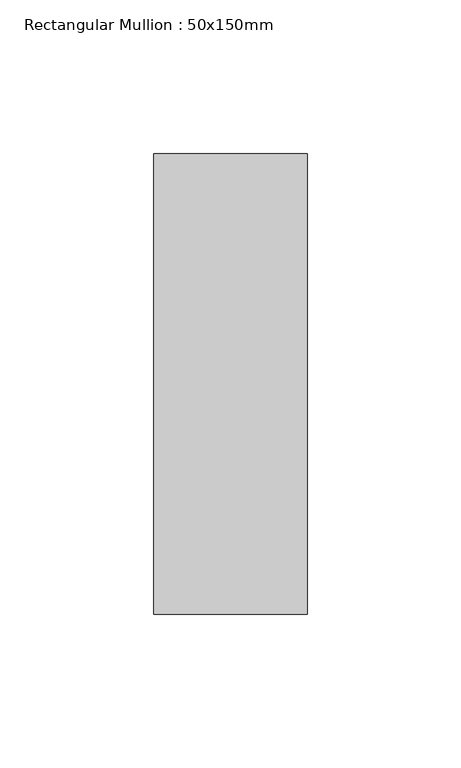
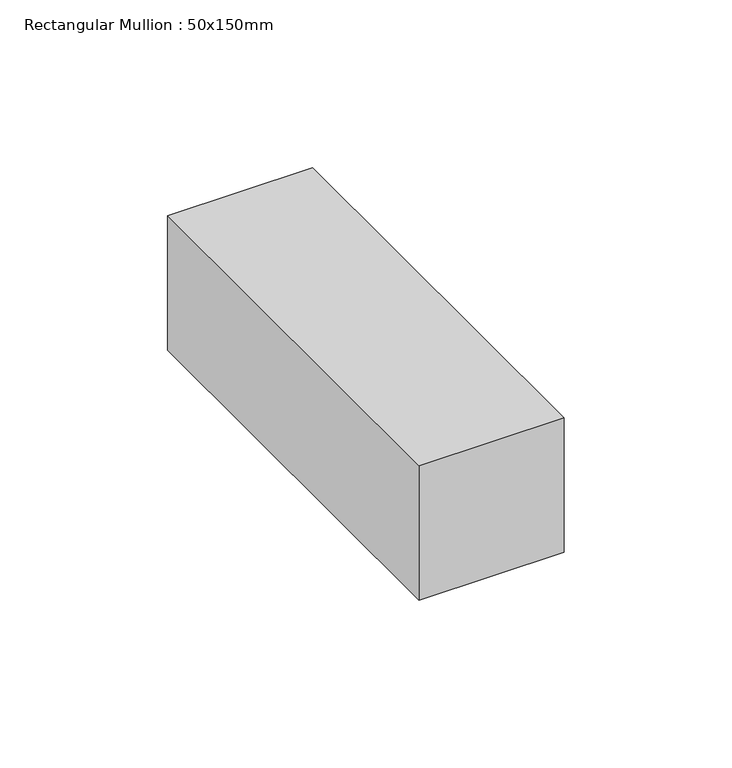
"""IFC4 building model written with IfcOpenShell, lengths in millimetres: member geometry, Rectangular Mullion : 50x150mm."""

from ifc_helpers import new_model, si_unit, frame, origin, place, context, project, spatial, polyline, outline, extrude, source, transform, mapped, element, save


def rectangular_mullion_50x150mm_fbc2abbf(model_context):
    return source(origin(), model_context, "Body", "SweptSolid", [
        extrude(outline(polyline([(25.0, 75.0), (25.0, -75.0), (-25.0, -75.0), (-25.0, 75.0), (25.0, 75.0)])), frame((0.0, 0.0, -49.0185145), z_axis=(0.0, 0.0, 1.0), x_axis=(1.0, 0.0, 0.0)), (0.0, 0.0, 1.0), 49.0185145),
    ])


if __name__ == "__main__":
    model = new_model("IFC4")
    model_context = context("Model", 3, world=origin())
    ifc_project = project(units=[si_unit("LENGTHUNIT", "METRE", prefix="MILLI")], contexts=[model_context])
    site = spatial("IfcSite", under=ifc_project)
    building = spatial("IfcBuilding", under=site)
    placement = place(None, origin())
    rectangular_mullion_50x150mm_shape = rectangular_mullion_50x150mm_fbc2abbf(model_context)
    element("IfcMember", 1, ObjectType="Rectangular Mullion : 50x150mm", at=placement, inside=building, context=model_context, shape_type="MappedRepresentation", body=[
        mapped(rectangular_mullion_50x150mm_shape, transform((0.0, 0.0, 0.0), x_axis=(1.0, 0.0, 0.0), y_axis=(0.0, 1.0, 0.0), z_axis=(0.0, 0.0, 1.0))),
    ])
    save(model, "model.ifc")

# Revit data of these elements
# Type "Rectangular Mullion : 50x150mm"
#   Keynote = "H11"
#   built-in parameter 1007304 = 0.492126 (stored number, unit not read)
#   built-in parameter 1007301 = 0.082021 (stored number, unit not read)
#   built-in parameter 1007300 = 0.082021 (stored number, unit not read)
# Element 1 (IfcMember, "Rectangular Mullion : 50x150mm")
#   Materials on its faces: "Aluminium"
# Materials
#   "Aluminium": class "Metal", colour RGB 247 247 247, transparency 0, Description = "Aluminium 6061", Cost = 0
